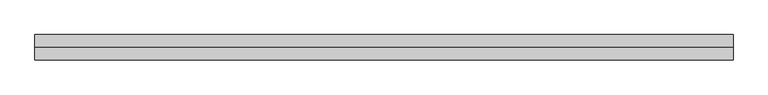
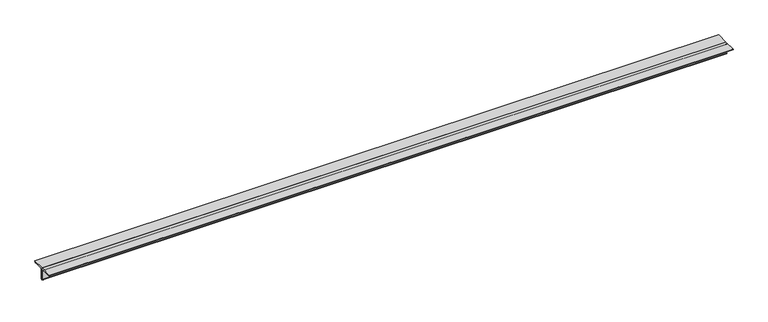
"""IFC4 building model written with IfcOpenShell, lengths in millimetres: member geometry, Steel Framing_2Ls_KS : H_SB_AR_S02_2Ls-100x100x10_VBR1."""

from ifc_helpers import new_model, si_unit, point, frame, frame_2d, origin, place, context, project, spatial, polyline, circle_curve, trimmed, segment, composite_curve, outline, extrude, source, transform, mapped, element, save


def member_0561801a(model_context):
    return source(origin(), model_context, "Body", "SweptSolid", [
        extrude(outline(composite_curve([segment(polyline([(0.0, 28.2), (0.0, -71.8)]), True, "CONTINUOUS"), segment(trimmed(circle_curve(frame_2d((0.0, -61.8)), 10.0), [point((0.0, -71.8))], [point((-10.0, -61.8))], False, "CARTESIAN"), True, "CONTINUOUS"), segment(polyline([(-10.0, -61.8), (-10.0, 8.2)]), True, "CONTINUOUS"), segment(trimmed(circle_curve(frame_2d((-20.0, 8.2)), 10.0), [point((-10.0, 8.2))], [point((-20.0, 18.2))], True, "CARTESIAN"), True, "CONTINUOUS"), segment(polyline([(-20.0, 18.2), (-90.0, 18.2)]), True, "CONTINUOUS"), segment(trimmed(circle_curve(frame_2d((-90.0, 28.2)), 10.0), [point((-90.0, 18.2))], [point((-100.0, 28.2))], False, "CARTESIAN"), True, "CONTINUOUS"), segment(polyline([(-100.0, 28.2), (0.0, 28.2)]), True, "CONTINUOUS")], self_intersect=False)), frame((-2590.3354834, 0.0, 0.0), z_axis=(1.0, 0.0, 0.0), x_axis=(0.0, 1.0, 0.0)), (0.0, 0.0, 1.0), 5505.8114308),
        extrude(outline(composite_curve([segment(polyline([(0.0, 28.2), (100.0, 28.2)]), True, "CONTINUOUS"), segment(trimmed(circle_curve(frame_2d((90.0, 28.2)), 10.0), [point((100.0, 28.2))], [point((90.0, 18.2))], False, "CARTESIAN"), True, "CONTINUOUS"), segment(polyline([(90.0, 18.2), (20.0, 18.2)]), True, "CONTINUOUS"), segment(trimmed(circle_curve(frame_2d((20.0, 8.2)), 10.0), [point((20.0, 18.2))], [point((10.0, 8.2))], True, "CARTESIAN"), True, "CONTINUOUS"), segment(polyline([(10.0, 8.2), (10.0, -61.8)]), True, "CONTINUOUS"), segment(trimmed(circle_curve(frame_2d((0.0, -61.8)), 10.0), [point((10.0, -61.8))], [point((0.0, -71.8))], False, "CARTESIAN"), True, "CONTINUOUS"), segment(polyline([(0.0, -71.8), (0.0, 28.2)]), True, "CONTINUOUS")], self_intersect=False)), frame((-2590.3354834, 0.0, 0.0), z_axis=(1.0, 0.0, 0.0), x_axis=(0.0, 1.0, 0.0)), (0.0, 0.0, 1.0), 5505.8114308),
    ])


if __name__ == "__main__":
    model = new_model("IFC4")
    model_context = context("Model", 3, world=origin())
    ifc_project = project(units=[si_unit("LENGTHUNIT", "METRE", prefix="MILLI")], contexts=[model_context])
    site = spatial("IfcSite", under=ifc_project)
    building = spatial("IfcBuilding", under=site)
    placement = place(None, origin())
    member_shape = member_0561801a(model_context)
    element("IfcMember", 1, ObjectType="Steel Framing_2Ls_KS : H_SB_AR_S02_2Ls-100x100x10_VBR1", at=placement, inside=building, context=model_context, shape_type="MappedRepresentation", body=[
        mapped(member_shape, transform((0.0, 0.0, 0.0), x_axis=(1.0, 0.0, 0.0), y_axis=(0.0, 1.0, 0.0), z_axis=(0.0, 0.0, 1.0))),
    ])
    save(model, "model.ifc")

# Revit data of these elements
# Type "Steel Framing_2Ls_KS : H_SB_AR_S02_2Ls-100x100x10_VBR1"
#   Type Comments = "MAIN"
#   Type Mark = "VBR1"
#   H_SectionID = "2Ls-100x100x10"
#   Assembly Code = "B10"
#   Legs = "LLBB"
#   H_Ratio for Additional Steel Plate = 0.2
#   W = 0
#   Perimeter = 0.80 m²/m
#   Nominal Weight = 29.80 kgf/m
#   Length [instance default] = 1524 mm
#   Space = 0 mm
#   b = 100 mm
#   d = 100 mm
#   t = 10 mm
#   y = 28.2 mm
#   A = 0.0038 m²
#   Structural Material [instance default] = Steel, 45-345
# Element 1 (IfcMember, "Steel Framing_2Ls_KS : H_SB_AR_S02_2Ls-100x100x10_VBR1")
#   Materials on its faces: "Steel, 45-345"
# Materials
#   "Steel, 45-345": class "Metal", colour RGB 189 187 185, transparency 0, Description = "Steel 345 MPa", Cost = 0
